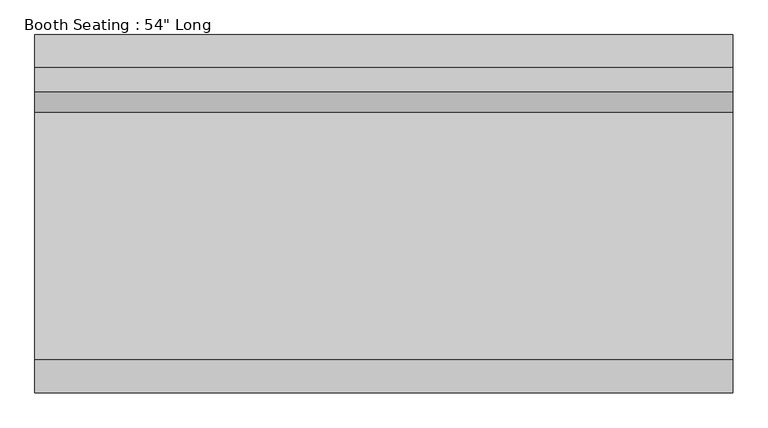
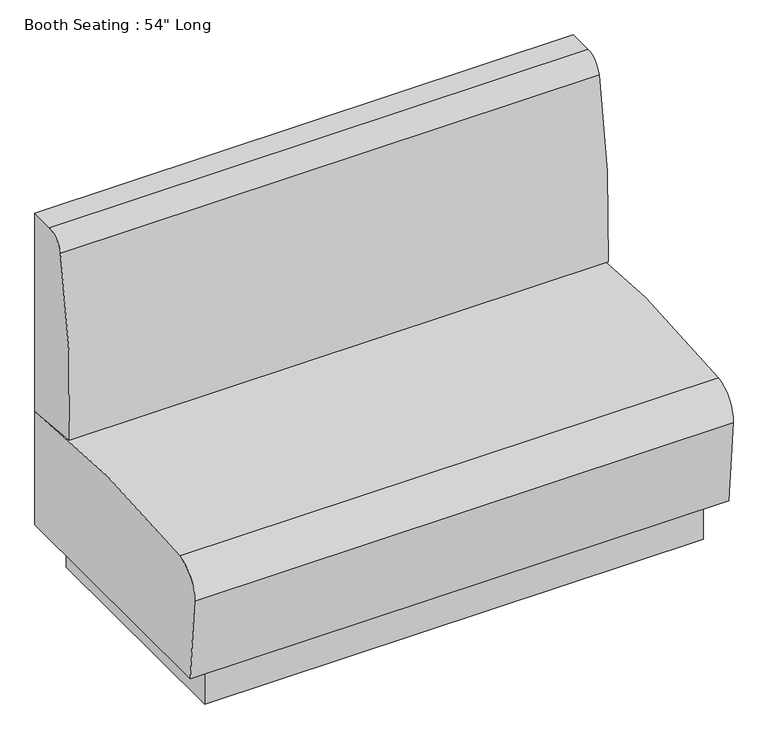
"""IFC4 building model written with IfcOpenShell, lengths in millimetres: furniture geometry."""

import ifcopenshell
import ifcopenshell.guid

model = None  # the IFC model being written
_history = None  # IfcOwnerHistory: only IFC2X3 demands one
_inside = {}  # id of a spatial element -> (the spatial element, [elements in it])
_under = {}  # id of a project, library or spatial element -> (it, [spatial elements below it])
_declared = {}  # id of a project -> (the project, [libraries it declares])
_typed = {}  # id of a type object -> (the type object, [elements of that type])
_made_of = {}  # id of a material, layer set ... -> (it, [elements and type objects made of it])


def new_model(schema):
    """Start an empty IFC model of exactly this schema.

    Asked for "IFC4X3", IfcOpenShell would pick the latest addendum, in which some entities
    have other attributes; the version numbers below select the first issue.
    IFC2X3 requires an IfcOwnerHistory on every rooted entity: one is made here for all.
    """
    global model, _history
    if schema == "IFC4X3":
        model = ifcopenshell.file(schema_version=(4, 3, 0, 0))
    else:
        model = ifcopenshell.file(schema=schema)
    _inside.clear()
    _under.clear()
    _declared.clear()
    _typed.clear()
    _made_of.clear()
    _history = None
    if model.schema == "IFC2X3":
        org = make("IfcOrganization", Name="unknown")
        user = make(
            "IfcPersonAndOrganization",
            ThePerson=make("IfcPerson", FamilyName="unknown"),
            TheOrganization=org,
        )
        app = make(
            "IfcApplication",
            ApplicationDeveloper=org,
            Version="unknown",
            ApplicationFullName="unknown",
            ApplicationIdentifier="unknown",
        )
        _history = make(
            "IfcOwnerHistory",
            OwningUser=user,
            OwningApplication=app,
            ChangeAction="ADDED",
            CreationDate=0,
        )
    return model


def make(cls, **values):
    """One entity of the class cls with the attributes given. An attribute that is None is left unset."""
    return model.create_entity(
        cls, **{name: value for name, value in values.items() if value is not None}
    )


def rooted(cls, **values):
    """An entity with a GlobalId (a new one), such as an element, a storey or a relation."""
    return make(cls, GlobalId=ifcopenshell.guid.new(), OwnerHistory=_history, **values)


def si_unit(unit_type, name, prefix=None):
    """IfcSIUnit, for example si_unit("LENGTHUNIT", "METRE", prefix="MILLI")."""
    return make("IfcSIUnit", UnitType=unit_type, Prefix=prefix, Name=name)


def assignment(units):
    """IfcUnitAssignment: the units of a project."""
    return None if units is None else make("IfcUnitAssignment", Units=units)


def point(xyz):
    """IfcCartesianPoint."""
    return None if xyz is None else make("IfcCartesianPoint", Coordinates=xyz)


def direction(xyz):
    """IfcDirection."""
    return None if xyz is None else make("IfcDirection", DirectionRatios=xyz)


def frame(location, z_axis=None, x_axis=None):
    """IfcAxis2Placement3D, a coordinate frame: its origin and axes. An axis left out is left unset."""
    return make(
        "IfcAxis2Placement3D",
        Location=point(location),
        Axis=direction(z_axis),
        RefDirection=direction(x_axis),
    )


def frame_2d(location, x_axis=None):
    """IfcAxis2Placement2D, a coordinate frame in the plane: its origin and x axis."""
    return make(
        "IfcAxis2Placement2D", Location=point(location), RefDirection=direction(x_axis)
    )


def origin():
    """The frame at (0, 0, 0) with its axes left unset."""
    return frame((0.0, 0.0, 0.0))


def origin_with_axes():
    """The frame at (0, 0, 0) with the z axis (0, 0, 1) and the x axis (1, 0, 0) written out."""
    return frame((0.0, 0.0, 0.0), z_axis=(0.0, 0.0, 1.0), x_axis=(1.0, 0.0, 0.0))


def place(relative_to, where):
    """IfcLocalPlacement: puts the frame where relative to a parent placement (None: the world)."""
    return make(
        "IfcLocalPlacement", PlacementRelTo=relative_to, RelativePlacement=where
    )


def context(
    kind, dimensions, precision=None, world=None, true_north=None, identifier=None
):
    """IfcGeometricRepresentationContext, for example the 3D "Model" context."""
    return make(
        "IfcGeometricRepresentationContext",
        ContextIdentifier=identifier,
        ContextType=kind,
        CoordinateSpaceDimension=dimensions,
        Precision=precision,
        WorldCoordinateSystem=world,
        TrueNorth=true_north,
    )


def project(units=None, contexts=None):
    """IfcProject with its units and contexts."""
    return rooted(
        "IfcProject",
        Name="project",
        RepresentationContexts=contexts,
        UnitsInContext=assignment(units),
    )


def spatial(cls, under=None, at=None, **own):
    """A site, building, storey or space (cls), placed at a placement, below another one or the project."""
    s = rooted(cls, ObjectPlacement=at, **own)
    if under is not None:
        _under.setdefault(under.id(), (under, []))[1].append(s)
    return s


def polyline(points):
    """IfcPolyline through the points."""
    return make("IfcPolyline", Points=[point(p) for p in points])


def circle_curve(where, radius):
    """IfcCircle in the frame where."""
    return make("IfcCircle", Position=where, Radius=radius)


def trimmed(basis, trim1, trim2, sense, master):
    """IfcTrimmedCurve: the piece of a basis curve between two trims."""
    return make(
        "IfcTrimmedCurve",
        BasisCurve=basis,
        Trim1=trim1,
        Trim2=trim2,
        SenseAgreement=sense,
        MasterRepresentation=master,
    )


def segment(curve, same_sense, transition):
    """IfcCompositeCurveSegment."""
    return make(
        "IfcCompositeCurveSegment",
        Transition=transition,
        SameSense=same_sense,
        ParentCurve=curve,
    )


def composite_curve(segments, self_intersect=None):
    """IfcCompositeCurve: segments joined end to end."""
    return make("IfcCompositeCurve", Segments=segments, SelfIntersect=self_intersect)


def outline(outer, holes=None, kind="AREA"):
    """IfcArbitraryClosedProfileDef: a profile drawn as a closed curve; with holes, ...WithVoids."""
    if holes is None:
        return make("IfcArbitraryClosedProfileDef", ProfileType=kind, OuterCurve=outer)
    return make(
        "IfcArbitraryProfileDefWithVoids",
        ProfileType=kind,
        OuterCurve=outer,
        InnerCurves=holes,
    )


def extrude(swept, where, along, depth):
    """IfcExtrudedAreaSolid: the profile swept, set in the frame where, extruded along a direction by depth."""
    return make(
        "IfcExtrudedAreaSolid",
        SweptArea=swept,
        Position=where,
        ExtrudedDirection=direction(along),
        Depth=depth,
    )


def shape(context_of_items, identifier, shape_type, items):
    """IfcShapeRepresentation: the items that make up one representation, for example the "Body"."""
    return make(
        "IfcShapeRepresentation",
        ContextOfItems=context_of_items,
        RepresentationIdentifier=identifier,
        RepresentationType=shape_type,
        Items=items,
    )


def source(mapping_origin, context_of_items, identifier, shape_type, items):
    """IfcRepresentationMap: a shape defined once, which mapped items show again and again."""
    return make(
        "IfcRepresentationMap",
        MappingOrigin=mapping_origin,
        MappedRepresentation=shape(context_of_items, identifier, shape_type, items),
    )


def transform(
    local_origin,
    x_axis=None,
    y_axis=None,
    z_axis=None,
    scale=None,
    scale2=None,
    scale3=None,
    uniform=True,
):
    """IfcCartesianTransformationOperator3D, or its non-uniform kind. x_axis, y_axis, z_axis: its Axis1, 2, 3."""
    if uniform:
        return make(
            "IfcCartesianTransformationOperator3D",
            Axis1=direction(x_axis),
            Axis2=direction(y_axis),
            LocalOrigin=point(local_origin),
            Scale=scale,
            Axis3=direction(z_axis),
        )
    return make(
        "IfcCartesianTransformationOperator3DnonUniform",
        Axis1=direction(x_axis),
        Axis2=direction(y_axis),
        LocalOrigin=point(local_origin),
        Scale=scale,
        Axis3=direction(z_axis),
        Scale2=scale2,
        Scale3=scale3,
    )


def mapped(mapping_source, mapping_target):
    """IfcMappedItem: shows the shape of a source again, moved by a transform."""
    return make(
        "IfcMappedItem", MappingSource=mapping_source, MappingTarget=mapping_target
    )


def made_of(thing, what):
    """Note that an element or type object is made of a material, layer set ...; save() writes the relation."""
    if what is not None:
        _made_of.setdefault(what.id(), (what, []))[1].append(thing)
    return thing


def element(
    cls,
    number,
    at=None,
    inside=None,
    cuts=None,
    type_object=None,
    material=None,
    context=None,
    identifier="Body",
    shape_type=None,
    held_by="IfcProductDefinitionShape",
    body=None,
    shapes=None,
    **own,
):
    """One element of the class cls, such as IfcWall. Its Tag is "e" and its number.

    at: its placement. inside: the storey or other place that contains it. cuts: it is an
    opening in that element (IfcRelVoidsElement). A single representation is given by context,
    identifier, shape_type and body (its items); several are given by shapes. held_by: the class
    of the entity that holds the representations. save() writes the other relations.
    """
    e = rooted(cls, Tag="e%d" % number, ObjectPlacement=at, **own)
    if body is not None:
        shapes = [shape(context, identifier, shape_type, body)]
    if shapes is not None:
        e.Representation = make(held_by, Representations=shapes)
    if inside is not None:
        _inside.setdefault(inside.id(), (inside, []))[1].append(e)
    if cuts is not None:
        rooted(
            "IfcRelVoidsElement", RelatingBuildingElement=cuts, RelatedOpeningElement=e
        )
    if type_object is not None:
        _typed.setdefault(type_object.id(), (type_object, []))[1].append(e)
    return made_of(e, material)


def aggregate(whole, parts):
    """IfcRelAggregates: a whole, such as a stair, and the parts it consists of."""
    return rooted("IfcRelAggregates", RelatingObject=whole, RelatedObjects=parts)


def save(model, path):
    """Write the relations noted so far, then the file.

    IfcRelAggregates (storeys below a building ...), IfcRelContainedInSpatialStructure (elements
    in a storey), IfcRelDefinesByType, IfcRelAssociatesMaterial and IfcRelDeclares: one each for
    every whole, place, type object, material and project.
    """
    for whole, parts in _under.values():
        aggregate(whole, parts)
    for where, things in _inside.values():
        rooted(
            "IfcRelContainedInSpatialStructure",
            RelatedElements=things,
            RelatingStructure=where,
        )
    for kind, things in _typed.values():
        rooted("IfcRelDefinesByType", RelatedObjects=things, RelatingType=kind)
    for what, things in _made_of.values():
        rooted("IfcRelAssociatesMaterial", RelatedObjects=things, RelatingMaterial=what)
    for by, libraries in _declared.values():
        rooted("IfcRelDeclares", RelatingContext=by, RelatedDefinitions=libraries)
    model.write(path)


def furniture_1a973976(model_context):
    return source(origin(), model_context, "Body", "SweptSolid", [
        extrude(outline(composite_curve([segment(polyline([(355.6, 939.8), (355.6, 406.4), (203.2, 420.809063)]), True, "CONTINUOUS"), segment(trimmed(circle_curve(frame_2d((1896.6191414, 522.5154157)), 1696.4706218), [point((203.2, 420.809063))], [point((242.7504703, 900.3129667))], False, "CARTESIAN"), True, "CONTINUOUS"), segment(trimmed(circle_curve(frame_2d((292.2747753, 889.0)), 50.8), [point((242.7504703, 900.3129667))], [point((292.2747753, 939.8))], False, "CARTESIAN"), True, "CONTINUOUS"), segment(polyline([(292.2747753, 939.8), (355.6, 939.8)]), True, "CONTINUOUS")], self_intersect=False)), frame((-685.8, 0.0, 0.0), z_axis=(1.0, 0.0, 0.0), x_axis=(0.0, 1.0, 0.0)), (0.0, 0.0, 1.0), 1371.6),
        extrude(outline(composite_curve([segment(trimmed(circle_curve(frame_2d((-272.6641824, 328.7396957)), 76.2), [point((-348.6009692, 322.4116302))], [point((-282.6626275, 404.2808838))], False, "CARTESIAN"), True, "CONTINUOUS"), segment(trimmed(circle_curve(frame_2d((44.6835428, -2068.9155338)), 2494.7657275), [point((-282.6626275, 404.2808838))], [point((355.6, 406.4))], False, "CARTESIAN"), True, "CONTINUOUS"), segment(polyline([(355.6, 406.4), (355.6, 101.6), (-330.2, 101.6), (-348.6009692, 322.4116302)]), True, "CONTINUOUS")], self_intersect=False)), frame((-685.8, 0.0, 0.0), z_axis=(1.0, 0.0, 0.0), x_axis=(0.0, 1.0, 0.0)), (0.0, 0.0, 1.0), 1371.6),
        extrude(outline(polyline([(635.0, 304.8), (635.0, -304.8), (-635.0, -304.8), (-635.0, 304.8), (635.0, 304.8)])), origin_with_axes(), (0.0, 0.0, 1.0), 101.6),
    ])


if __name__ == "__main__":
    model = new_model("IFC4")
    model_context = context("Model", 3, world=origin())
    ifc_project = project(units=[si_unit("LENGTHUNIT", "METRE", prefix="MILLI")], contexts=[model_context])
    site = spatial("IfcSite", under=ifc_project)
    building = spatial("IfcBuilding", under=site)
    placement = place(None, origin())
    furniture_shape = furniture_1a973976(model_context)
    element("IfcFurniture", 1, ObjectType="Booth Seating : 54\" Long", at=placement, inside=building, context=model_context, shape_type="MappedRepresentation", body=[
        mapped(furniture_shape, transform((0.0, 0.0, 0.0), x_axis=(1.0, 0.0, 0.0), y_axis=(0.0, 1.0, 0.0), z_axis=(0.0, 0.0, 1.0))),
    ])
    save(model, "model.ifc")

# Revit data of these elements
# Project information
#   Project Issue Date = "Issue Date"
#   Project Status = "Project Status"
#   Client Name = "Owner"
#   Project Address = "Enter address here"
#   Project Name = "Project Name"
#   Project Number = "Project Number"
# Type "Booth Seating : 54\" Long"
#   Seat Height = 1' - 4"
#   Length = 4' - 6"
#   Depth = 2' - 4"
#   Back Height = 3' - 1"
#   Default Elevation = 0
# Element 1 (IfcFurniture, "Booth Seating : 54\" Long")
#   Materials on its faces: "Leather, Dark Brown", "Plastic, Opaque Black"
# Materials
#   "Leather, Dark Brown": class "Textile", colour RGB 57 45 39, transparency 0, Description = "Leather, dark brown", Cost = 0
#   "Plastic, Opaque Black": class "Plastic", colour RGB 5 5 5, transparency 0, Description = "Plastic, generic, opaque black", Cost = 0
